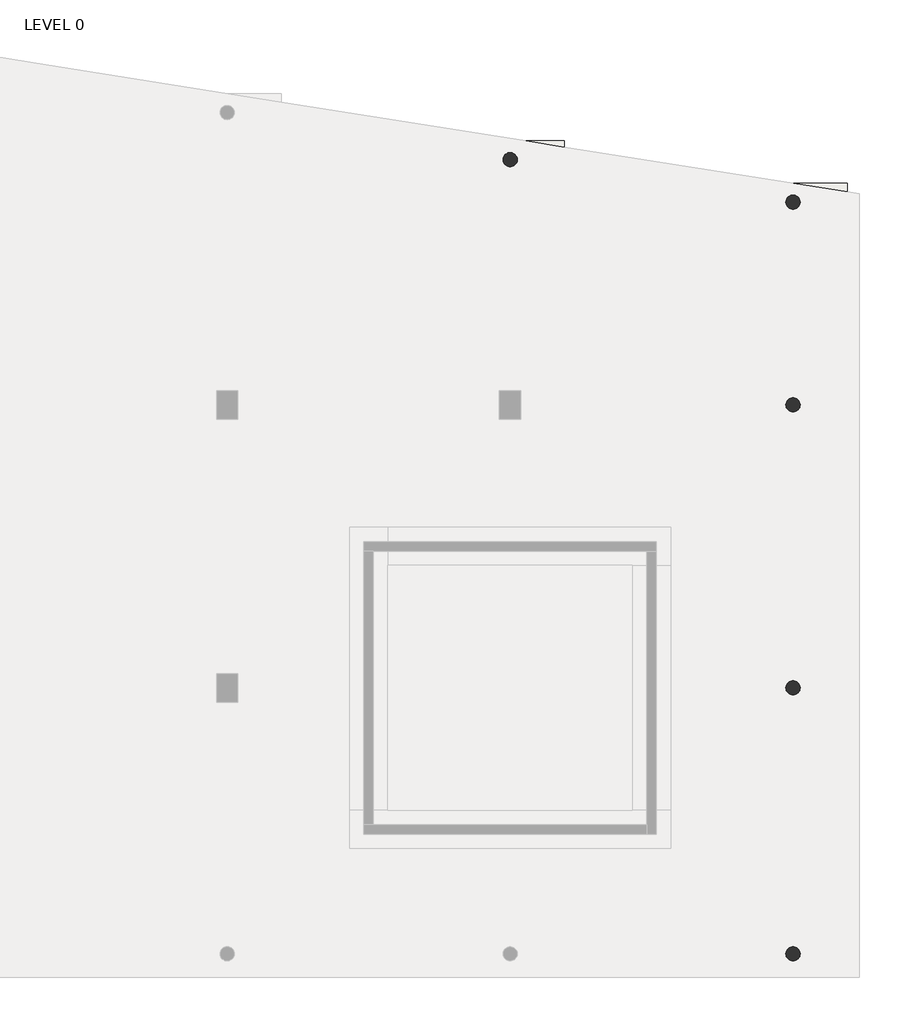
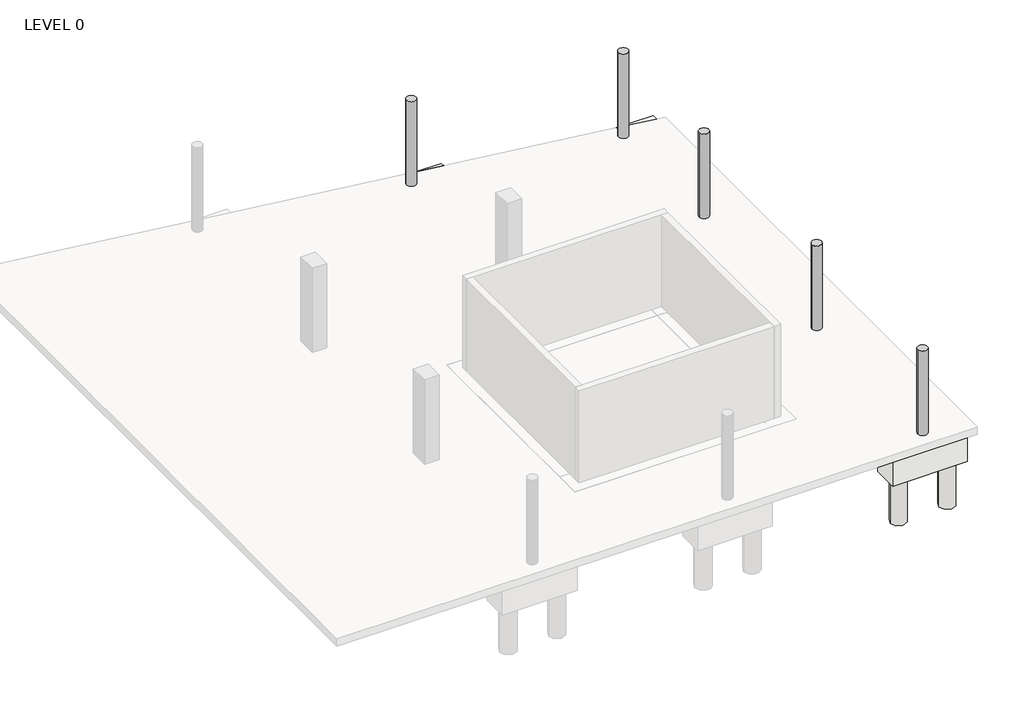
# One storey, part 3 of 3: 17 slabs, 5 columns.
"""IFC4 building model written with IfcOpenShell, lengths in millimetres."""

from ifc_helpers import new_model, si_unit, point, frame, frame_2d, origin, origin_with_axes, place, context, project, spatial, polyline, circle_curve, trimmed, segment, composite_curve, outline, extrude, element, save
from ifc_brep_helpers import plane_surface, cylinder_surface, revolved_surface, advanced_brep

model = new_model("IFC4")

# Units and contexts
model_context = context("Model", 3, world=origin())
ifc_project = project(units=[si_unit("LENGTHUNIT", "METRE", prefix="MILLI")], contexts=[model_context])

# Site, building, storey
site = spatial("IfcSite", under=ifc_project)
building = spatial("IfcBuilding", under=site)
storey = spatial("IfcBuildingStorey", under=building, Name="LEVEL 0", Elevation=0.0)

# Columns
placement = place(None, origin())
element("IfcColumn", 1, ObjectType="BHm_StructuralColumns_ConcreteRound : 300 Ø RC COL", at=placement, inside=storey, context=model_context, shape_type="SweptSolid", body=[
    extrude(outline(composite_curve([segment(trimmed(circle_curve(frame_2d((924.8319731, 14640.7845261)), 150.0), [point((774.8319731, 14640.7845261))], [point((1074.8319731, 14640.7845261))], False, "CARTESIAN"), True, "CONTINUOUS"), segment(trimmed(circle_curve(frame_2d((924.8319731, 14640.7845261)), 150.0), [point((1074.8319731, 14640.7845261))], [point((774.8319731, 14640.7845261))], False, "CARTESIAN"), True, "CONTINUOUS")], self_intersect=False)), origin_with_axes(), (0.0, 0.0, 1.0), 2750.0),
])
element("IfcColumn", 2, ObjectType="BHm_StructuralColumns_ConcreteRound : 300 Ø RC COL", at=placement, inside=storey, context=model_context, shape_type="SweptSolid", body=[
    extrude(outline(composite_curve([segment(trimmed(circle_curve(frame_2d((924.8319731, 8640.7845261)), 150.0), [point((774.8319731, 8640.7845261))], [point((1074.8319731, 8640.7845261))], False, "CARTESIAN"), True, "CONTINUOUS"), segment(trimmed(circle_curve(frame_2d((924.8319731, 8640.7845261)), 150.0), [point((1074.8319731, 8640.7845261))], [point((774.8319731, 8640.7845261))], False, "CARTESIAN"), True, "CONTINUOUS")], self_intersect=False)), origin_with_axes(), (0.0, 0.0, 1.0), 2750.0),
])
element("IfcColumn", 3, ObjectType="BHm_StructuralColumns_ConcreteRound : 300 Ø RC COL", at=placement, inside=storey, context=model_context, shape_type="SweptSolid", body=[
    extrude(outline(composite_curve([segment(trimmed(circle_curve(frame_2d((924.8319731, 3000.0)), 150.0), [point((774.8319731, 3000.0))], [point((1074.8319731, 3000.0))], False, "CARTESIAN"), True, "CONTINUOUS"), segment(trimmed(circle_curve(frame_2d((924.8319731, 3000.0)), 150.0), [point((1074.8319731, 3000.0))], [point((774.8319731, 3000.0))], False, "CARTESIAN"), True, "CONTINUOUS")], self_intersect=False)), origin_with_axes(), (0.0, 0.0, 1.0), 2750.0),
])
element("IfcColumn", 4, ObjectType="BHm_StructuralColumns_ConcreteRound : 300 Ø RC COL", at=placement, inside=storey, context=model_context, shape_type="SweptSolid", body=[
    extrude(outline(composite_curve([segment(trimmed(circle_curve(frame_2d((-5075.1680269, 19840.7845261)), 150.0), [point((-5225.1680269, 19840.7845261))], [point((-4925.1680269, 19840.7845261))], False, "CARTESIAN"), True, "CONTINUOUS"), segment(trimmed(circle_curve(frame_2d((-5075.1680269, 19840.7845261)), 150.0), [point((-4925.1680269, 19840.7845261))], [point((-5225.1680269, 19840.7845261))], False, "CARTESIAN"), True, "CONTINUOUS")], self_intersect=False)), origin_with_axes(), (0.0, 0.0, 1.0), 2750.0),
])
element("IfcColumn", 5, ObjectType="BHm_StructuralColumns_ConcreteRound : 300 Ø RC COL", at=placement, inside=storey, context=model_context, shape_type="SweptSolid", body=[
    extrude(outline(composite_curve([segment(trimmed(circle_curve(frame_2d((924.8319731, 18940.7845261)), 150.0), [point((774.8319731, 18940.7845261))], [point((1074.8319731, 18940.7845261))], False, "CARTESIAN"), True, "CONTINUOUS"), segment(trimmed(circle_curve(frame_2d((924.8319731, 18940.7845261)), 150.0), [point((1074.8319731, 18940.7845261))], [point((774.8319731, 18940.7845261))], False, "CARTESIAN"), True, "CONTINUOUS")], self_intersect=False)), origin_with_axes(), (0.0, 0.0, 1.0), 2750.0),
])

# Slabs
element("IfcSlab", 6, ObjectType="BHm_StructuralFoundations_RC-2PileCap : 500Ø R.C. 2-PILE CAP", at=placement, inside=storey, context=model_context, shape_type="AdvancedBrep", body=[
    advanced_brep(
    [(2074.8319731, 3400.0, -1100.0), (2074.8319731, 2600.0, -1100.0), (-225.1680269, 2600.0, -1100.0), (-225.1680269, 3400.0, -1100.0), (-75.1680269, 3000.0, -1100.0), (424.8319731, 3000.0, -1100.0), (1424.8319731, 3000.0, -1100.0), (1924.8319731, 3000.0, -1100.0), (-225.1680269, 3400.0, -250.0), (2074.8319731, 3400.0, -250.0), (-225.1680269, 2600.0, -250.0), (2074.8319731, 2600.0, -250.0), (1424.8319731, 3000.0, -1025.0), (1924.8319731, 3000.0, -1025.0), (-75.1680269, 3000.0, -1025.0), (424.8319731, 3000.0, -1025.0)],
    [
        (0, 1),
        (1, 2),
        (2, 3),
        (3, 0),
        (4, 5, circle_curve(frame((174.8319731, 3000.0, -1100.0), z_axis=(0.0, 0.0, 1.0), x_axis=(1.0, 0.0, 0.0)), 250.0)),
        (5, 4, circle_curve(frame((174.8319731, 3000.0, -1100.0), z_axis=(0.0, 0.0, 1.0), x_axis=(1.0, 0.0, 0.0)), 250.0)),
        (6, 7, circle_curve(frame((1674.8319731, 3000.0, -1100.0), z_axis=(0.0, 0.0, 1.0), x_axis=(1.0, 0.0, 0.0)), 250.0)),
        (7, 6, circle_curve(frame((1674.8319731, 3000.0, -1100.0), z_axis=(0.0, 0.0, 1.0), x_axis=(1.0, 0.0, 0.0)), 250.0)),
        (3, 8),
        (8, 9),
        (9, 0),
        (2, 10),
        (10, 8),
        (1, 11),
        (11, 10),
        (9, 11),
        (12, 13, circle_curve(frame((1674.8319731, 3000.0, -1025.0), z_axis=(0.0, 0.0, -1.0), x_axis=(1.0, 0.0, 0.0)), 250.0)),
        (13, 12, circle_curve(frame((1674.8319731, 3000.0, -1025.0), z_axis=(0.0, 0.0, -1.0), x_axis=(1.0, 0.0, 0.0)), 250.0)),
        (4, 14),
        (14, 15, circle_curve(frame((174.8319731, 3000.0, -1025.0), z_axis=(0.0, 0.0, 1.0), x_axis=(1.0, 0.0, 0.0)), 250.0)),
        (15, 5),
        (15, 14, circle_curve(frame((174.8319731, 3000.0, -1025.0), z_axis=(0.0, 0.0, 1.0), x_axis=(1.0, 0.0, 0.0)), 250.0)),
        (6, 12),
        (13, 7),
    ],
    [
        plane_surface(frame((-225.1680269, 3400.0, -1100.0), z_axis=(0.0, 0.0, -1.0), x_axis=(1.0, 0.0, 0.0))),
        plane_surface(frame((2074.8319731, 3400.0, 0.0), z_axis=(0.0, 1.0, 0.0), x_axis=(0.0, 0.0, -1.0))),
        plane_surface(frame((-225.1680269, 3400.0, 0.0), z_axis=(-1.0, 0.0, 0.0), x_axis=(0.0, 0.0, -1.0))),
        plane_surface(frame((-225.1680269, 2600.0, 0.0), z_axis=(0.0, -1.0, 0.0), x_axis=(0.0, 0.0, -1.0))),
        plane_surface(frame((2074.8319731, 2600.0, 0.0), z_axis=(1.0, 0.0, 0.0), x_axis=(0.0, 0.0, -1.0))),
        plane_surface(frame((424.8319731, 3000.0, -1025.0), z_axis=(0.0, 0.0, -1.0), x_axis=(0.0, 1.0, 0.0))),
        revolved_surface(polyline([(424.8319731, 3000.0, -1025.0), (424.8319731, 3000.0, -1100.0)]), (174.8319731, 3000.0, -1100.0), (0.0, 0.0, 1.0)),
        revolved_surface(polyline([(1924.8319731, 3000.0, -1025.0), (1924.8319731, 3000.0, -1100.0)]), (1674.8319731, 3000.0, 0.0), (0.0, 0.0, 1.0)),
        plane_surface(frame((2324.8319731, 15140.7845261, -250.0), z_axis=(0.0, 0.0, 1.0), x_axis=(0.0, -1.0, 0.0))),
    ],
    [
        (0, [[1, 2, 3, 4], [5, 6], [7, 8]]),
        (1, [[-4, 9, 10, 11]]),
        (2, [[-3, 12, 13, -9]]),
        (3, [[-2, 14, 15, -12]]),
        (4, [[-1, -11, 16, -14]]),
        (5, [[17, 18]]),
        (6, [[-5, 19, 20, 21]]),
        (6, [[-6, -21, 22, -19]]),
        (7, [[-7, 23, -18, 24]]),
        (7, [[-8, -24, -17, -23]]),
        (8, [[-10, -13, -15, -16]]),
        (5, [[-22, -20]]),
    ],
),
])
element("IfcSlab", 7, ObjectType="BHm_StructuralFoundations_RC-Pile : 500Ø R.C. PILE", at=placement, inside=storey, context=model_context, shape_type="AdvancedBrep", body=[
    advanced_brep(
    [(-75.1680269, 3000.0, -1025.0), (424.8319731, 3000.0, -1025.0), (-75.1680269, 3000.0, -2600.0), (424.8319731, 3000.0, -2600.0), (-75.1680269, 3000.0, -1100.0), (424.8319731, 3000.0, -1100.0)],
    [
        (0, 1, circle_curve(frame((174.8319731, 3000.0, -1025.0), z_axis=(0.0, 0.0, 1.0), x_axis=(1.0, 0.0, 0.0)), 250.0)),
        (1, 0, circle_curve(frame((174.8319731, 3000.0, -1025.0), z_axis=(0.0, 0.0, 1.0), x_axis=(1.0, 0.0, 0.0)), 250.0)),
        (2, 3, circle_curve(frame((174.8319731, 3000.0, -2600.0), z_axis=(0.0, 0.0, -1.0), x_axis=(1.0, 0.0, 0.0)), 250.0)),
        (3, 2, circle_curve(frame((174.8319731, 3000.0, -2600.0), z_axis=(0.0, 0.0, -1.0), x_axis=(1.0, 0.0, 0.0)), 250.0)),
        (0, 4),
        (4, 2),
        (3, 5),
        (5, 1),
    ],
    [
        plane_surface(frame((424.8319731, 3000.0, -1025.0), z_axis=(0.0, 0.0, 1.0), x_axis=(0.0, 1.0, 0.0))),
        plane_surface(frame((424.8319731, 3000.0, -2600.0), z_axis=(0.0, 0.0, -1.0), x_axis=(0.0, -1.0, 0.0))),
        cylinder_surface(frame((174.8319731, 3000.0, -2600.0), z_axis=(0.0, 0.0, 1.0), x_axis=(1.0, 0.0, 0.0)), 250.0),
    ],
    [
        (0, [[1, 2]]),
        (1, [[3, 4]]),
        (2, [[-1, 5, 6, -4, 7, 8]]),
        (2, [[-2, -8, -7, -3, -6, -5]]),
    ],
),
])
element("IfcSlab", 8, ObjectType="BHm_StructuralFoundations_RC-Pile : 500Ø R.C. PILE", at=placement, inside=storey, context=model_context, shape_type="AdvancedBrep", body=[
    advanced_brep(
    [(1424.8319731, 3000.0, -1025.0), (1924.8319731, 3000.0, -1025.0), (1424.8319731, 3000.0, -2600.0), (1924.8319731, 3000.0, -2600.0), (1424.8319731, 3000.0, -1100.0), (1924.8319731, 3000.0, -1100.0)],
    [
        (0, 1, circle_curve(frame((1674.8319731, 3000.0, -1025.0), z_axis=(0.0, 0.0, 1.0), x_axis=(1.0, 0.0, 0.0)), 250.0)),
        (1, 0, circle_curve(frame((1674.8319731, 3000.0, -1025.0), z_axis=(0.0, 0.0, 1.0), x_axis=(1.0, 0.0, 0.0)), 250.0)),
        (2, 3, circle_curve(frame((1674.8319731, 3000.0, -2600.0), z_axis=(0.0, 0.0, -1.0), x_axis=(1.0, 0.0, 0.0)), 250.0)),
        (3, 2, circle_curve(frame((1674.8319731, 3000.0, -2600.0), z_axis=(0.0, 0.0, -1.0), x_axis=(1.0, 0.0, 0.0)), 250.0)),
        (0, 4),
        (4, 2),
        (3, 5),
        (5, 1),
    ],
    [
        plane_surface(frame((1924.8319731, 3000.0, -1025.0), z_axis=(0.0, 0.0, 1.0), x_axis=(0.0, 1.0, 0.0))),
        plane_surface(frame((1924.8319731, 3000.0, -2600.0), z_axis=(0.0, 0.0, -1.0), x_axis=(0.0, -1.0, 0.0))),
        cylinder_surface(frame((1674.8319731, 3000.0, -2600.0), z_axis=(0.0, 0.0, 1.0), x_axis=(1.0, 0.0, 0.0)), 250.0),
    ],
    [
        (0, [[1, 2]]),
        (1, [[3, 4]]),
        (2, [[-1, 5, 6, -4, 7, 8]]),
        (2, [[-2, -8, -7, -3, -6, -5]]),
    ],
),
])
element("IfcSlab", 9, ObjectType="BHm_StructuralFoundations_RC-2PileCap : 500Ø R.C. 2-PILE CAP", at=placement, inside=storey, context=model_context, shape_type="AdvancedBrep", body=[
    advanced_brep(
    [(2074.8319731, 9040.7845261, -1100.0), (2074.8319731, 8240.7845261, -1100.0), (-225.1680269, 8240.7845261, -1100.0), (-225.1680269, 9040.7845261, -1100.0), (-75.1680269, 8640.7845261, -1100.0), (424.8319731, 8640.7845261, -1100.0), (1424.8319731, 8640.7845261, -1100.0), (1924.8319731, 8640.7845261, -1100.0), (-225.1680269, 9040.7845261, -250.0), (2074.8319731, 9040.7845261, -250.0), (-225.1680269, 8240.7845261, -250.0), (2074.8319731, 8240.7845261, -250.0), (1424.8319731, 8640.7845261, -1025.0), (1924.8319731, 8640.7845261, -1025.0), (-75.1680269, 8640.7845261, -1025.0), (424.8319731, 8640.7845261, -1025.0)],
    [
        (0, 1),
        (1, 2),
        (2, 3),
        (3, 0),
        (4, 5, circle_curve(frame((174.8319731, 8640.7845261, -1100.0), z_axis=(0.0, 0.0, 1.0), x_axis=(1.0, 0.0, 0.0)), 250.0)),
        (5, 4, circle_curve(frame((174.8319731, 8640.7845261, -1100.0), z_axis=(0.0, 0.0, 1.0), x_axis=(1.0, 0.0, 0.0)), 250.0)),
        (6, 7, circle_curve(frame((1674.8319731, 8640.7845261, -1100.0), z_axis=(0.0, 0.0, 1.0), x_axis=(1.0, 0.0, 0.0)), 250.0)),
        (7, 6, circle_curve(frame((1674.8319731, 8640.7845261, -1100.0), z_axis=(0.0, 0.0, 1.0), x_axis=(1.0, 0.0, 0.0)), 250.0)),
        (3, 8),
        (8, 9),
        (9, 0),
        (2, 10),
        (10, 8),
        (1, 11),
        (11, 10),
        (9, 11),
        (12, 13, circle_curve(frame((1674.8319731, 8640.7845261, -1025.0), z_axis=(0.0, 0.0, -1.0), x_axis=(1.0, 0.0, 0.0)), 250.0)),
        (13, 12, circle_curve(frame((1674.8319731, 8640.7845261, -1025.0), z_axis=(0.0, 0.0, -1.0), x_axis=(1.0, 0.0, 0.0)), 250.0)),
        (4, 14),
        (14, 15, circle_curve(frame((174.8319731, 8640.7845261, -1025.0), z_axis=(0.0, 0.0, 1.0), x_axis=(1.0, 0.0, 0.0)), 250.0)),
        (15, 5),
        (15, 14, circle_curve(frame((174.8319731, 8640.7845261, -1025.0), z_axis=(0.0, 0.0, 1.0), x_axis=(1.0, 0.0, 0.0)), 250.0)),
        (6, 12),
        (13, 7),
    ],
    [
        plane_surface(frame((-225.1680269, 9040.7845261, -1100.0), z_axis=(0.0, 0.0, -1.0), x_axis=(1.0, 0.0, 0.0))),
        plane_surface(frame((2074.8319731, 9040.7845261, 0.0), z_axis=(0.0, 1.0, 0.0), x_axis=(0.0, 0.0, -1.0))),
        plane_surface(frame((-225.1680269, 9040.7845261, 0.0), z_axis=(-1.0, 0.0, 0.0), x_axis=(0.0, 0.0, -1.0))),
        plane_surface(frame((-225.1680269, 8240.7845261, 0.0), z_axis=(0.0, -1.0, 0.0), x_axis=(0.0, 0.0, -1.0))),
        plane_surface(frame((2074.8319731, 8240.7845261, 0.0), z_axis=(1.0, 0.0, 0.0), x_axis=(0.0, 0.0, -1.0))),
        plane_surface(frame((424.8319731, 8640.7845261, -1025.0), z_axis=(0.0, 0.0, -1.0), x_axis=(0.0, 1.0, 0.0))),
        revolved_surface(polyline([(424.8319731, 8640.7845261, -1025.0), (424.8319731, 8640.7845261, -1100.0)]), (174.8319731, 8640.7845261, -1100.0), (0.0, 0.0, 1.0)),
        revolved_surface(polyline([(1924.8319731, 8640.7845261, -1025.0), (1924.8319731, 8640.7845261, -1100.0)]), (1674.8319731, 8640.7845261, 0.0), (0.0, 0.0, 1.0)),
        plane_surface(frame((2324.8319731, 15140.7845261, -250.0), z_axis=(0.0, 0.0, 1.0), x_axis=(0.0, -1.0, 0.0))),
    ],
    [
        (0, [[1, 2, 3, 4], [5, 6], [7, 8]]),
        (1, [[-4, 9, 10, 11]]),
        (2, [[-3, 12, 13, -9]]),
        (3, [[-2, 14, 15, -12]]),
        (4, [[-1, -11, 16, -14]]),
        (5, [[17, 18]]),
        (6, [[-5, 19, 20, 21]]),
        (6, [[-6, -21, 22, -19]]),
        (7, [[-7, 23, -18, 24]]),
        (7, [[-8, -24, -17, -23]]),
        (8, [[-10, -13, -15, -16]]),
        (5, [[-22, -20]]),
    ],
),
])
element("IfcSlab", 10, ObjectType="BHm_StructuralFoundations_RC-Pile : 500Ø R.C. PILE", at=placement, inside=storey, context=model_context, shape_type="AdvancedBrep", body=[
    advanced_brep(
    [(-75.1680269, 8640.7845261, -1025.0), (424.8319731, 8640.7845261, -1025.0), (-75.1680269, 8640.7845261, -2600.0), (424.8319731, 8640.7845261, -2600.0), (-75.1680269, 8640.7845261, -1100.0), (424.8319731, 8640.7845261, -1100.0)],
    [
        (0, 1, circle_curve(frame((174.8319731, 8640.7845261, -1025.0), z_axis=(0.0, 0.0, 1.0), x_axis=(1.0, 0.0, 0.0)), 250.0)),
        (1, 0, circle_curve(frame((174.8319731, 8640.7845261, -1025.0), z_axis=(0.0, 0.0, 1.0), x_axis=(1.0, 0.0, 0.0)), 250.0)),
        (2, 3, circle_curve(frame((174.8319731, 8640.7845261, -2600.0), z_axis=(0.0, 0.0, -1.0), x_axis=(1.0, 0.0, 0.0)), 250.0)),
        (3, 2, circle_curve(frame((174.8319731, 8640.7845261, -2600.0), z_axis=(0.0, 0.0, -1.0), x_axis=(1.0, 0.0, 0.0)), 250.0)),
        (0, 4),
        (4, 2),
        (3, 5),
        (5, 1),
    ],
    [
        plane_surface(frame((424.8319731, 8640.7845261, -1025.0), z_axis=(0.0, 0.0, 1.0), x_axis=(0.0, 1.0, 0.0))),
        plane_surface(frame((424.8319731, 8640.7845261, -2600.0), z_axis=(0.0, 0.0, -1.0), x_axis=(0.0, -1.0, 0.0))),
        cylinder_surface(frame((174.8319731, 8640.7845261, -2600.0), z_axis=(0.0, 0.0, 1.0), x_axis=(1.0, 0.0, 0.0)), 250.0),
    ],
    [
        (0, [[1, 2]]),
        (1, [[3, 4]]),
        (2, [[-1, 5, 6, -4, 7, 8]]),
        (2, [[-2, -8, -7, -3, -6, -5]]),
    ],
),
])
element("IfcSlab", 11, ObjectType="BHm_StructuralFoundations_RC-Pile : 500Ø R.C. PILE", at=placement, inside=storey, context=model_context, shape_type="AdvancedBrep", body=[
    advanced_brep(
    [(1424.8319731, 8640.7845261, -1025.0), (1924.8319731, 8640.7845261, -1025.0), (1424.8319731, 8640.7845261, -2600.0), (1924.8319731, 8640.7845261, -2600.0), (1424.8319731, 8640.7845261, -1100.0), (1924.8319731, 8640.7845261, -1100.0)],
    [
        (0, 1, circle_curve(frame((1674.8319731, 8640.7845261, -1025.0), z_axis=(0.0, 0.0, 1.0), x_axis=(1.0, 0.0, 0.0)), 250.0)),
        (1, 0, circle_curve(frame((1674.8319731, 8640.7845261, -1025.0), z_axis=(0.0, 0.0, 1.0), x_axis=(1.0, 0.0, 0.0)), 250.0)),
        (2, 3, circle_curve(frame((1674.8319731, 8640.7845261, -2600.0), z_axis=(0.0, 0.0, -1.0), x_axis=(1.0, 0.0, 0.0)), 250.0)),
        (3, 2, circle_curve(frame((1674.8319731, 8640.7845261, -2600.0), z_axis=(0.0, 0.0, -1.0), x_axis=(1.0, 0.0, 0.0)), 250.0)),
        (0, 4),
        (4, 2),
        (3, 5),
        (5, 1),
    ],
    [
        plane_surface(frame((1924.8319731, 8640.7845261, -1025.0), z_axis=(0.0, 0.0, 1.0), x_axis=(0.0, 1.0, 0.0))),
        plane_surface(frame((1924.8319731, 8640.7845261, -2600.0), z_axis=(0.0, 0.0, -1.0), x_axis=(0.0, -1.0, 0.0))),
        cylinder_surface(frame((1674.8319731, 8640.7845261, -2600.0), z_axis=(0.0, 0.0, 1.0), x_axis=(1.0, 0.0, 0.0)), 250.0),
    ],
    [
        (0, [[1, 2]]),
        (1, [[3, 4]]),
        (2, [[-1, 5, 6, -4, 7, 8]]),
        (2, [[-2, -8, -7, -3, -6, -5]]),
    ],
),
])
element("IfcSlab", 12, ObjectType="BHm_StructuralFoundations_RC-2PileCap : 500Ø R.C. 2-PILE CAP", at=placement, inside=storey, context=model_context, shape_type="AdvancedBrep", body=[
    advanced_brep(
    [(2074.8319731, 15040.7845261, -1100.0), (2074.8319731, 14240.7845261, -1100.0), (-225.1680269, 14240.7845261, -1100.0), (-225.1680269, 15040.7845261, -1100.0), (-75.1680269, 14640.7845261, -1100.0), (424.8319731, 14640.7845261, -1100.0), (1424.8319731, 14640.7845261, -1100.0), (1924.8319731, 14640.7845261, -1100.0), (-225.1680269, 15040.7845261, -250.0), (2074.8319731, 15040.7845261, -250.0), (-225.1680269, 14240.7845261, -250.0), (2074.8319731, 14240.7845261, -250.0), (1424.8319731, 14640.7845261, -1025.0), (1924.8319731, 14640.7845261, -1025.0), (-75.1680269, 14640.7845261, -1025.0), (424.8319731, 14640.7845261, -1025.0)],
    [
        (0, 1),
        (1, 2),
        (2, 3),
        (3, 0),
        (4, 5, circle_curve(frame((174.8319731, 14640.7845261, -1100.0), z_axis=(0.0, 0.0, 1.0), x_axis=(1.0, 0.0, 0.0)), 250.0)),
        (5, 4, circle_curve(frame((174.8319731, 14640.7845261, -1100.0), z_axis=(0.0, 0.0, 1.0), x_axis=(1.0, 0.0, 0.0)), 250.0)),
        (6, 7, circle_curve(frame((1674.8319731, 14640.7845261, -1100.0), z_axis=(0.0, 0.0, 1.0), x_axis=(1.0, 0.0, 0.0)), 250.0)),
        (7, 6, circle_curve(frame((1674.8319731, 14640.7845261, -1100.0), z_axis=(0.0, 0.0, 1.0), x_axis=(1.0, 0.0, 0.0)), 250.0)),
        (3, 8),
        (8, 9),
        (9, 0),
        (2, 10),
        (10, 8),
        (1, 11),
        (11, 10),
        (9, 11),
        (12, 13, circle_curve(frame((1674.8319731, 14640.7845261, -1025.0), z_axis=(0.0, 0.0, -1.0), x_axis=(1.0, 0.0, 0.0)), 250.0)),
        (13, 12, circle_curve(frame((1674.8319731, 14640.7845261, -1025.0), z_axis=(0.0, 0.0, -1.0), x_axis=(1.0, 0.0, 0.0)), 250.0)),
        (4, 14),
        (14, 15, circle_curve(frame((174.8319731, 14640.7845261, -1025.0), z_axis=(0.0, 0.0, 1.0), x_axis=(1.0, 0.0, 0.0)), 250.0)),
        (15, 5),
        (15, 14, circle_curve(frame((174.8319731, 14640.7845261, -1025.0), z_axis=(0.0, 0.0, 1.0), x_axis=(1.0, 0.0, 0.0)), 250.0)),
        (6, 12),
        (13, 7),
    ],
    [
        plane_surface(frame((-225.1680269, 15040.7845261, -1100.0), z_axis=(0.0, 0.0, -1.0), x_axis=(1.0, 0.0, 0.0))),
        plane_surface(frame((2074.8319731, 15040.7845261, 0.0), z_axis=(0.0, 1.0, 0.0), x_axis=(0.0, 0.0, -1.0))),
        plane_surface(frame((-225.1680269, 15040.7845261, 0.0), z_axis=(-1.0, 0.0, 0.0), x_axis=(0.0, 0.0, -1.0))),
        plane_surface(frame((-225.1680269, 14240.7845261, 0.0), z_axis=(0.0, -1.0, 0.0), x_axis=(0.0, 0.0, -1.0))),
        plane_surface(frame((2074.8319731, 14240.7845261, 0.0), z_axis=(1.0, 0.0, 0.0), x_axis=(0.0, 0.0, -1.0))),
        plane_surface(frame((424.8319731, 14640.7845261, -1025.0), z_axis=(0.0, 0.0, -1.0), x_axis=(0.0, 1.0, 0.0))),
        revolved_surface(polyline([(424.8319731, 14640.7845261, -1025.0), (424.8319731, 14640.7845261, -1100.0)]), (174.8319731, 14640.7845261, -1100.0), (0.0, 0.0, 1.0)),
        revolved_surface(polyline([(1924.8319731, 14640.7845261, -1025.0), (1924.8319731, 14640.7845261, -1100.0)]), (1674.8319731, 14640.7845261, 0.0), (0.0, 0.0, 1.0)),
        plane_surface(frame((2324.8319731, 15140.7845261, -250.0), z_axis=(0.0, 0.0, 1.0), x_axis=(0.0, -1.0, 0.0))),
    ],
    [
        (0, [[1, 2, 3, 4], [5, 6], [7, 8]]),
        (1, [[-4, 9, 10, 11]]),
        (2, [[-3, 12, 13, -9]]),
        (3, [[-2, 14, 15, -12]]),
        (4, [[-1, -11, 16, -14]]),
        (5, [[17, 18]]),
        (6, [[-5, 19, 20, 21]]),
        (6, [[-6, -21, 22, -19]]),
        (7, [[-7, 23, -18, 24]]),
        (7, [[-8, -24, -17, -23]]),
        (8, [[-10, -13, -15, -16]]),
        (5, [[-22, -20]]),
    ],
),
])
element("IfcSlab", 13, ObjectType="BHm_StructuralFoundations_RC-Pile : 500Ø R.C. PILE", at=placement, inside=storey, context=model_context, shape_type="AdvancedBrep", body=[
    advanced_brep(
    [(-75.1680269, 14640.7845261, -1025.0), (424.8319731, 14640.7845261, -1025.0), (-75.1680269, 14640.7845261, -2600.0), (424.8319731, 14640.7845261, -2600.0), (-75.1680269, 14640.7845261, -1100.0), (424.8319731, 14640.7845261, -1100.0)],
    [
        (0, 1, circle_curve(frame((174.8319731, 14640.7845261, -1025.0), z_axis=(0.0, 0.0, 1.0), x_axis=(1.0, 0.0, 0.0)), 250.0)),
        (1, 0, circle_curve(frame((174.8319731, 14640.7845261, -1025.0), z_axis=(0.0, 0.0, 1.0), x_axis=(1.0, 0.0, 0.0)), 250.0)),
        (2, 3, circle_curve(frame((174.8319731, 14640.7845261, -2600.0), z_axis=(0.0, 0.0, -1.0), x_axis=(1.0, 0.0, 0.0)), 250.0)),
        (3, 2, circle_curve(frame((174.8319731, 14640.7845261, -2600.0), z_axis=(0.0, 0.0, -1.0), x_axis=(1.0, 0.0, 0.0)), 250.0)),
        (0, 4),
        (4, 2),
        (3, 5),
        (5, 1),
    ],
    [
        plane_surface(frame((424.8319731, 14640.7845261, -1025.0), z_axis=(0.0, 0.0, 1.0), x_axis=(0.0, 1.0, 0.0))),
        plane_surface(frame((424.8319731, 14640.7845261, -2600.0), z_axis=(0.0, 0.0, -1.0), x_axis=(0.0, -1.0, 0.0))),
        cylinder_surface(frame((174.8319731, 14640.7845261, -2600.0), z_axis=(0.0, 0.0, 1.0), x_axis=(1.0, 0.0, 0.0)), 250.0),
    ],
    [
        (0, [[1, 2]]),
        (1, [[3, 4]]),
        (2, [[-1, 5, 6, -4, 7, 8]]),
        (2, [[-2, -8, -7, -3, -6, -5]]),
    ],
),
])
element("IfcSlab", 14, ObjectType="BHm_StructuralFoundations_RC-Pile : 500Ø R.C. PILE", at=placement, inside=storey, context=model_context, shape_type="AdvancedBrep", body=[
    advanced_brep(
    [(1424.8319731, 14640.7845261, -1025.0), (1924.8319731, 14640.7845261, -1025.0), (1424.8319731, 14640.7845261, -2600.0), (1924.8319731, 14640.7845261, -2600.0), (1424.8319731, 14640.7845261, -1100.0), (1924.8319731, 14640.7845261, -1100.0)],
    [
        (0, 1, circle_curve(frame((1674.8319731, 14640.7845261, -1025.0), z_axis=(0.0, 0.0, 1.0), x_axis=(1.0, 0.0, 0.0)), 250.0)),
        (1, 0, circle_curve(frame((1674.8319731, 14640.7845261, -1025.0), z_axis=(0.0, 0.0, 1.0), x_axis=(1.0, 0.0, 0.0)), 250.0)),
        (2, 3, circle_curve(frame((1674.8319731, 14640.7845261, -2600.0), z_axis=(0.0, 0.0, -1.0), x_axis=(1.0, 0.0, 0.0)), 250.0)),
        (3, 2, circle_curve(frame((1674.8319731, 14640.7845261, -2600.0), z_axis=(0.0, 0.0, -1.0), x_axis=(1.0, 0.0, 0.0)), 250.0)),
        (0, 4),
        (4, 2),
        (3, 5),
        (5, 1),
    ],
    [
        plane_surface(frame((1924.8319731, 14640.7845261, -1025.0), z_axis=(0.0, 0.0, 1.0), x_axis=(0.0, 1.0, 0.0))),
        plane_surface(frame((1924.8319731, 14640.7845261, -2600.0), z_axis=(0.0, 0.0, -1.0), x_axis=(0.0, -1.0, 0.0))),
        cylinder_surface(frame((1674.8319731, 14640.7845261, -2600.0), z_axis=(0.0, 0.0, 1.0), x_axis=(1.0, 0.0, 0.0)), 250.0),
    ],
    [
        (0, [[1, 2]]),
        (1, [[3, 4]]),
        (2, [[-1, 5, 6, -4, 7, 8]]),
        (2, [[-2, -8, -7, -3, -6, -5]]),
    ],
),
])
element("IfcSlab", 15, ObjectType="BHm_StructuralFoundations_RC-Pile : 500Ø R.C. PILE", at=placement, inside=storey, context=model_context, shape_type="AdvancedBrep", body=[
    advanced_brep(
    [(-12075.1680269, 20840.7845261, -1025.0), (-11575.1680269, 20840.7845261, -1025.0), (-12075.1680269, 20840.7845261, -2600.0), (-11575.1680269, 20840.7845261, -2600.0), (-12075.1680269, 20840.7845261, -1100.0), (-11575.1680269, 20840.7845261, -1100.0)],
    [
        (0, 1, circle_curve(frame((-11825.1680269, 20840.7845261, -1025.0), z_axis=(0.0, 0.0, 1.0), x_axis=(1.0, 0.0, 0.0)), 250.0)),
        (1, 0, circle_curve(frame((-11825.1680269, 20840.7845261, -1025.0), z_axis=(0.0, 0.0, 1.0), x_axis=(1.0, 0.0, 0.0)), 250.0)),
        (2, 3, circle_curve(frame((-11825.1680269, 20840.7845261, -2600.0), z_axis=(0.0, 0.0, -1.0), x_axis=(1.0, 0.0, 0.0)), 250.0)),
        (3, 2, circle_curve(frame((-11825.1680269, 20840.7845261, -2600.0), z_axis=(0.0, 0.0, -1.0), x_axis=(1.0, 0.0, 0.0)), 250.0)),
        (0, 4),
        (4, 2),
        (3, 5),
        (5, 1),
    ],
    [
        plane_surface(frame((-11575.1680269, 20840.7845261, -1025.0), z_axis=(0.0, 0.0, 1.0), x_axis=(0.0, 1.0, 0.0))),
        plane_surface(frame((-11575.1680269, 20840.7845261, -2600.0), z_axis=(0.0, 0.0, -1.0), x_axis=(0.0, -1.0, 0.0))),
        cylinder_surface(frame((-11825.1680269, 20840.7845261, -2600.0), z_axis=(0.0, 0.0, 1.0), x_axis=(1.0, 0.0, 0.0)), 250.0),
    ],
    [
        (0, [[1, 2]]),
        (1, [[3, 4]]),
        (2, [[-1, 5, 6, -4, 7, 8]]),
        (2, [[-2, -8, -7, -3, -6, -5]]),
    ],
),
])
element("IfcSlab", 16, ObjectType="BHm_StructuralFoundations_RC-Pile : 500Ø R.C. PILE", at=placement, inside=storey, context=model_context, shape_type="AdvancedBrep", body=[
    advanced_brep(
    [(-10575.1680269, 20840.7845261, -1025.0), (-10075.1680269, 20840.7845261, -1025.0), (-10575.1680269, 20840.7845261, -2600.0), (-10075.1680269, 20840.7845261, -2600.0), (-10575.1680269, 20840.7845261, -1100.0), (-10075.1680269, 20840.7845261, -1100.0)],
    [
        (0, 1, circle_curve(frame((-10325.1680269, 20840.7845261, -1025.0), z_axis=(0.0, 0.0, 1.0), x_axis=(1.0, 0.0, 0.0)), 250.0)),
        (1, 0, circle_curve(frame((-10325.1680269, 20840.7845261, -1025.0), z_axis=(0.0, 0.0, 1.0), x_axis=(1.0, 0.0, 0.0)), 250.0)),
        (2, 3, circle_curve(frame((-10325.1680269, 20840.7845261, -2600.0), z_axis=(0.0, 0.0, -1.0), x_axis=(1.0, 0.0, 0.0)), 250.0)),
        (3, 2, circle_curve(frame((-10325.1680269, 20840.7845261, -2600.0), z_axis=(0.0, 0.0, -1.0), x_axis=(1.0, 0.0, 0.0)), 250.0)),
        (0, 4),
        (4, 2),
        (3, 5),
        (5, 1),
    ],
    [
        plane_surface(frame((-10075.1680269, 20840.7845261, -1025.0), z_axis=(0.0, 0.0, 1.0), x_axis=(0.0, 1.0, 0.0))),
        plane_surface(frame((-10075.1680269, 20840.7845261, -2600.0), z_axis=(0.0, 0.0, -1.0), x_axis=(0.0, -1.0, 0.0))),
        cylinder_surface(frame((-10325.1680269, 20840.7845261, -2600.0), z_axis=(0.0, 0.0, 1.0), x_axis=(1.0, 0.0, 0.0)), 250.0),
    ],
    [
        (0, [[1, 2]]),
        (1, [[3, 4]]),
        (2, [[-1, 5, 6, -4, 7, 8]]),
        (2, [[-2, -8, -7, -3, -6, -5]]),
    ],
),
])
element("IfcSlab", 17, ObjectType="BHm_StructuralFoundations_RC-2PileCap : 500Ø R.C. 2-PILE CAP", at=placement, inside=storey, context=model_context, shape_type="AdvancedBrep", body=[
    advanced_brep(
    [(-3925.1680269, 20240.7845261, 0.0), (-4747.6649976, 20240.7845261, 0.0), (-3925.1680269, 20110.5138037, 0.0), (-3925.1680269, 20240.7845261, -1100.0), (-3925.1680269, 19440.7845261, -1100.0), (-6225.1680269, 19440.7845261, -1100.0), (-6225.1680269, 20240.7845261, -1100.0), (-6075.1680269, 19840.7845261, -1100.0), (-5575.1680269, 19840.7845261, -1100.0), (-4575.1680269, 19840.7845261, -1100.0), (-4075.1680269, 19840.7845261, -1100.0), (-6225.1680269, 20240.7845261, -250.0), (-4747.6649976, 20240.7845261, -250.0), (-6225.1680269, 19440.7845261, -250.0), (-3925.1680269, 19440.7845261, -250.0), (-3925.1680269, 20110.5138037, -250.0), (-4575.1680269, 19840.7845261, -1025.0), (-4075.1680269, 19840.7845261, -1025.0), (-6075.1680269, 19840.7845261, -1025.0), (-5575.1680269, 19840.7845261, -1025.0)],
    [
        (0, 1),
        (1, 2),
        (2, 0),
        (3, 4),
        (4, 5),
        (5, 6),
        (6, 3),
        (7, 8, circle_curve(frame((-5825.1680269, 19840.7845261, -1100.0), z_axis=(0.0, 0.0, 1.0), x_axis=(1.0, 0.0, 0.0)), 250.0)),
        (8, 7, circle_curve(frame((-5825.1680269, 19840.7845261, -1100.0), z_axis=(0.0, 0.0, 1.0), x_axis=(1.0, 0.0, 0.0)), 250.0)),
        (9, 10, circle_curve(frame((-4325.1680269, 19840.7845261, -1100.0), z_axis=(0.0, 0.0, 1.0), x_axis=(1.0, 0.0, 0.0)), 250.0)),
        (10, 9, circle_curve(frame((-4325.1680269, 19840.7845261, -1100.0), z_axis=(0.0, 0.0, 1.0), x_axis=(1.0, 0.0, 0.0)), 250.0)),
        (6, 11),
        (11, 12),
        (12, 1),
        (0, 3),
        (5, 13),
        (13, 11),
        (4, 14),
        (14, 13),
        (2, 15),
        (15, 14),
        (16, 17, circle_curve(frame((-4325.1680269, 19840.7845261, -1025.0), z_axis=(0.0, 0.0, -1.0), x_axis=(1.0, 0.0, 0.0)), 250.0)),
        (17, 16, circle_curve(frame((-4325.1680269, 19840.7845261, -1025.0), z_axis=(0.0, 0.0, -1.0), x_axis=(1.0, 0.0, 0.0)), 250.0)),
        (7, 18),
        (18, 19, circle_curve(frame((-5825.1680269, 19840.7845261, -1025.0), z_axis=(0.0, 0.0, 1.0), x_axis=(1.0, 0.0, 0.0)), 250.0)),
        (19, 8),
        (19, 18, circle_curve(frame((-5825.1680269, 19840.7845261, -1025.0), z_axis=(0.0, 0.0, 1.0), x_axis=(1.0, 0.0, 0.0)), 250.0)),
        (9, 16),
        (17, 10),
        (15, 12),
    ],
    [
        plane_surface(frame((-6225.1680269, 20240.7845261, 0.0), z_axis=(0.0, 0.0, 1.0), x_axis=(-1.0, 0.0, 0.0))),
        plane_surface(frame((-6225.1680269, 20240.7845261, -1100.0), z_axis=(0.0, 0.0, -1.0), x_axis=(1.0, 0.0, 0.0))),
        plane_surface(frame((-3925.1680269, 20240.7845261, 0.0), z_axis=(0.0, 1.0, 0.0), x_axis=(0.0, 0.0, -1.0))),
        plane_surface(frame((-6225.1680269, 20240.7845261, 0.0), z_axis=(-1.0, 0.0, 0.0), x_axis=(0.0, 0.0, -1.0))),
        plane_surface(frame((-6225.1680269, 19440.7845261, 0.0), z_axis=(0.0, -1.0, 0.0), x_axis=(0.0, 0.0, -1.0))),
        plane_surface(frame((-3925.1680269, 19440.7845261, 0.0), z_axis=(1.0, 0.0, 0.0), x_axis=(0.0, 0.0, -1.0))),
        plane_surface(frame((-5575.1680269, 19840.7845261, -1025.0), z_axis=(0.0, 0.0, -1.0), x_axis=(0.0, 1.0, 0.0))),
        revolved_surface(polyline([(-5575.1680269, 19840.7845261, -1025.0), (-5575.1680269, 19840.7845261, -1100.0)]), (-5825.1680269, 19840.7845261, -1100.0), (0.0, 0.0, 1.0)),
        revolved_surface(polyline([(-4075.1680269, 19840.7845261, -1025.0), (-4075.1680269, 19840.7845261, -1100.0)]), (-4325.1680269, 19840.7845261, 0.0), (0.0, 0.0, 1.0)),
        plane_surface(frame((2324.8319731, 15140.7845261, -250.0), z_axis=(0.0, 0.0, 1.0), x_axis=(0.0, -1.0, 0.0))),
        plane_surface(frame((-17375.1680269, 22240.7845261, -250.0), z_axis=(-0.15643446504023414, -0.9876883405951372, 0.0), x_axis=(0.0, 0.0, 1.0))),
    ],
    [
        (0, [[1, 2, 3]]),
        (1, [[4, 5, 6, 7], [8, 9], [10, 11]]),
        (2, [[-7, 12, 13, 14, -1, 15]]),
        (3, [[-6, 16, 17, -12]]),
        (4, [[-5, 18, 19, -16]]),
        (5, [[-4, -15, -3, 20, 21, -18]]),
        (6, [[22, 23]]),
        (7, [[-8, 24, 25, 26]]),
        (7, [[-9, -26, 27, -24]]),
        (8, [[-10, 28, -23, 29]]),
        (8, [[-11, -29, -22, -28]]),
        (9, [[30, -13, -17, -19, -21]]),
        (10, [[-30, -20, -2, -14]]),
        (6, [[-27, -25]]),
    ],
),
])
element("IfcSlab", 18, ObjectType="BHm_StructuralFoundations_RC-Pile : 500Ø R.C. PILE", at=placement, inside=storey, context=model_context, shape_type="AdvancedBrep", body=[
    advanced_brep(
    [(-6075.1680269, 19840.7845261, -1025.0), (-5575.1680269, 19840.7845261, -1025.0), (-6075.1680269, 19840.7845261, -2600.0), (-5575.1680269, 19840.7845261, -2600.0), (-6075.1680269, 19840.7845261, -1100.0), (-5575.1680269, 19840.7845261, -1100.0)],
    [
        (0, 1, circle_curve(frame((-5825.1680269, 19840.7845261, -1025.0), z_axis=(0.0, 0.0, 1.0), x_axis=(1.0, 0.0, 0.0)), 250.0)),
        (1, 0, circle_curve(frame((-5825.1680269, 19840.7845261, -1025.0), z_axis=(0.0, 0.0, 1.0), x_axis=(1.0, 0.0, 0.0)), 250.0)),
        (2, 3, circle_curve(frame((-5825.1680269, 19840.7845261, -2600.0), z_axis=(0.0, 0.0, -1.0), x_axis=(1.0, 0.0, 0.0)), 250.0)),
        (3, 2, circle_curve(frame((-5825.1680269, 19840.7845261, -2600.0), z_axis=(0.0, 0.0, -1.0), x_axis=(1.0, 0.0, 0.0)), 250.0)),
        (0, 4),
        (4, 2),
        (3, 5),
        (5, 1),
    ],
    [
        plane_surface(frame((-5575.1680269, 19840.7845261, -1025.0), z_axis=(0.0, 0.0, 1.0), x_axis=(0.0, 1.0, 0.0))),
        plane_surface(frame((-5575.1680269, 19840.7845261, -2600.0), z_axis=(0.0, 0.0, -1.0), x_axis=(0.0, -1.0, 0.0))),
        cylinder_surface(frame((-5825.1680269, 19840.7845261, -2600.0), z_axis=(0.0, 0.0, 1.0), x_axis=(1.0, 0.0, 0.0)), 250.0),
    ],
    [
        (0, [[1, 2]]),
        (1, [[3, 4]]),
        (2, [[-1, 5, 6, -4, 7, 8]]),
        (2, [[-2, -8, -7, -3, -6, -5]]),
    ],
),
])
element("IfcSlab", 19, ObjectType="BHm_StructuralFoundations_RC-Pile : 500Ø R.C. PILE", at=placement, inside=storey, context=model_context, shape_type="AdvancedBrep", body=[
    advanced_brep(
    [(-4575.1680269, 19840.7845261, -1025.0), (-4075.1680269, 19840.7845261, -1025.0), (-4575.1680269, 19840.7845261, -2600.0), (-4075.1680269, 19840.7845261, -2600.0), (-4575.1680269, 19840.7845261, -1100.0), (-4075.1680269, 19840.7845261, -1100.0)],
    [
        (0, 1, circle_curve(frame((-4325.1680269, 19840.7845261, -1025.0), z_axis=(0.0, 0.0, 1.0), x_axis=(1.0, 0.0, 0.0)), 250.0)),
        (1, 0, circle_curve(frame((-4325.1680269, 19840.7845261, -1025.0), z_axis=(0.0, 0.0, 1.0), x_axis=(1.0, 0.0, 0.0)), 250.0)),
        (2, 3, circle_curve(frame((-4325.1680269, 19840.7845261, -2600.0), z_axis=(0.0, 0.0, -1.0), x_axis=(1.0, 0.0, 0.0)), 250.0)),
        (3, 2, circle_curve(frame((-4325.1680269, 19840.7845261, -2600.0), z_axis=(0.0, 0.0, -1.0), x_axis=(1.0, 0.0, 0.0)), 250.0)),
        (0, 4),
        (4, 2),
        (3, 5),
        (5, 1),
    ],
    [
        plane_surface(frame((-4075.1680269, 19840.7845261, -1025.0), z_axis=(0.0, 0.0, 1.0), x_axis=(0.0, 1.0, 0.0))),
        plane_surface(frame((-4075.1680269, 19840.7845261, -2600.0), z_axis=(0.0, 0.0, -1.0), x_axis=(0.0, -1.0, 0.0))),
        cylinder_surface(frame((-4325.1680269, 19840.7845261, -2600.0), z_axis=(0.0, 0.0, 1.0), x_axis=(1.0, 0.0, 0.0)), 250.0),
    ],
    [
        (0, [[1, 2]]),
        (1, [[3, 4]]),
        (2, [[-1, 5, 6, -4, 7, 8]]),
        (2, [[-2, -8, -7, -3, -6, -5]]),
    ],
),
])
element("IfcSlab", 20, ObjectType="BHm_StructuralFoundations_RC-2PileCap : 500Ø R.C. 2-PILE CAP", at=placement, inside=storey, context=model_context, shape_type="AdvancedBrep", body=[
    advanced_brep(
    [(2074.8319731, 19340.7845261, 0.0), (934.7113656, 19340.7845261, 0.0), (2074.8319731, 19160.2071617, 0.0), (2074.8319731, 19340.7845261, -1100.0), (2074.8319731, 18540.7845261, -1100.0), (-225.1680269, 18540.7845261, -1100.0), (-225.1680269, 19340.7845261, -1100.0), (-75.1680269, 18940.7845261, -1100.0), (424.8319731, 18940.7845261, -1100.0), (1424.8319731, 18940.7845261, -1100.0), (1924.8319731, 18940.7845261, -1100.0), (-225.1680269, 19340.7845261, -250.0), (934.7113656, 19340.7845261, -250.0), (-225.1680269, 18540.7845261, -250.0), (2074.8319731, 18540.7845261, -250.0), (2074.8319731, 19160.2071617, -250.0), (1424.8319731, 18940.7845261, -1025.0), (1924.8319731, 18940.7845261, -1025.0), (-75.1680269, 18940.7845261, -1025.0), (424.8319731, 18940.7845261, -1025.0)],
    [
        (0, 1),
        (1, 2),
        (2, 0),
        (3, 4),
        (4, 5),
        (5, 6),
        (6, 3),
        (7, 8, circle_curve(frame((174.8319731, 18940.7845261, -1100.0), z_axis=(0.0, 0.0, 1.0), x_axis=(1.0, 0.0, 0.0)), 250.0)),
        (8, 7, circle_curve(frame((174.8319731, 18940.7845261, -1100.0), z_axis=(0.0, 0.0, 1.0), x_axis=(1.0, 0.0, 0.0)), 250.0)),
        (9, 10, circle_curve(frame((1674.8319731, 18940.7845261, -1100.0), z_axis=(0.0, 0.0, 1.0), x_axis=(1.0, 0.0, 0.0)), 250.0)),
        (10, 9, circle_curve(frame((1674.8319731, 18940.7845261, -1100.0), z_axis=(0.0, 0.0, 1.0), x_axis=(1.0, 0.0, 0.0)), 250.0)),
        (6, 11),
        (11, 12),
        (12, 1),
        (0, 3),
        (5, 13),
        (13, 11),
        (4, 14),
        (14, 13),
        (2, 15),
        (15, 14),
        (16, 17, circle_curve(frame((1674.8319731, 18940.7845261, -1025.0), z_axis=(0.0, 0.0, -1.0), x_axis=(1.0, 0.0, 0.0)), 250.0)),
        (17, 16, circle_curve(frame((1674.8319731, 18940.7845261, -1025.0), z_axis=(0.0, 0.0, -1.0), x_axis=(1.0, 0.0, 0.0)), 250.0)),
        (7, 18),
        (18, 19, circle_curve(frame((174.8319731, 18940.7845261, -1025.0), z_axis=(0.0, 0.0, 1.0), x_axis=(1.0, 0.0, 0.0)), 250.0)),
        (19, 8),
        (19, 18, circle_curve(frame((174.8319731, 18940.7845261, -1025.0), z_axis=(0.0, 0.0, 1.0), x_axis=(1.0, 0.0, 0.0)), 250.0)),
        (9, 16),
        (17, 10),
        (15, 12),
    ],
    [
        plane_surface(frame((-225.1680269, 19340.7845261, 0.0), z_axis=(0.0, 0.0, 1.0), x_axis=(-1.0, 0.0, 0.0))),
        plane_surface(frame((-225.1680269, 19340.7845261, -1100.0), z_axis=(0.0, 0.0, -1.0), x_axis=(1.0, 0.0, 0.0))),
        plane_surface(frame((2074.8319731, 19340.7845261, 0.0), z_axis=(0.0, 1.0, 0.0), x_axis=(0.0, 0.0, -1.0))),
        plane_surface(frame((-225.1680269, 19340.7845261, 0.0), z_axis=(-1.0, 0.0, 0.0), x_axis=(0.0, 0.0, -1.0))),
        plane_surface(frame((-225.1680269, 18540.7845261, 0.0), z_axis=(0.0, -1.0, 0.0), x_axis=(0.0, 0.0, -1.0))),
        plane_surface(frame((2074.8319731, 18540.7845261, 0.0), z_axis=(1.0, 0.0, 0.0), x_axis=(0.0, 0.0, -1.0))),
        plane_surface(frame((424.8319731, 18940.7845261, -1025.0), z_axis=(0.0, 0.0, -1.0), x_axis=(0.0, 1.0, 0.0))),
        revolved_surface(polyline([(424.8319731, 18940.7845261, -1025.0), (424.8319731, 18940.7845261, -1100.0)]), (174.8319731, 18940.7845261, -1100.0), (0.0, 0.0, 1.0)),
        revolved_surface(polyline([(1924.8319731, 18940.7845261, -1025.0), (1924.8319731, 18940.7845261, -1100.0)]), (1674.8319731, 18940.7845261, 0.0), (0.0, 0.0, 1.0)),
        plane_surface(frame((2324.8319731, 15140.7845261, -250.0), z_axis=(0.0, 0.0, 1.0), x_axis=(0.0, -1.0, 0.0))),
        plane_surface(frame((-17375.1680269, 22240.7845261, -250.0), z_axis=(-0.15643446504023414, -0.9876883405951372, 0.0), x_axis=(0.0, 0.0, 1.0))),
    ],
    [
        (0, [[1, 2, 3]]),
        (1, [[4, 5, 6, 7], [8, 9], [10, 11]]),
        (2, [[-7, 12, 13, 14, -1, 15]]),
        (3, [[-6, 16, 17, -12]]),
        (4, [[-5, 18, 19, -16]]),
        (5, [[-4, -15, -3, 20, 21, -18]]),
        (6, [[22, 23]]),
        (7, [[-8, 24, 25, 26]]),
        (7, [[-9, -26, 27, -24]]),
        (8, [[-10, 28, -23, 29]]),
        (8, [[-11, -29, -22, -28]]),
        (9, [[30, -13, -17, -19, -21]]),
        (10, [[-30, -20, -2, -14]]),
        (6, [[-27, -25]]),
    ],
),
])
element("IfcSlab", 21, ObjectType="BHm_StructuralFoundations_RC-Pile : 500Ø R.C. PILE", at=placement, inside=storey, context=model_context, shape_type="AdvancedBrep", body=[
    advanced_brep(
    [(-75.1680269, 18940.7845261, -1025.0), (424.8319731, 18940.7845261, -1025.0), (-75.1680269, 18940.7845261, -2600.0), (424.8319731, 18940.7845261, -2600.0), (-75.1680269, 18940.7845261, -1100.0), (424.8319731, 18940.7845261, -1100.0)],
    [
        (0, 1, circle_curve(frame((174.8319731, 18940.7845261, -1025.0), z_axis=(0.0, 0.0, 1.0), x_axis=(1.0, 0.0, 0.0)), 250.0)),
        (1, 0, circle_curve(frame((174.8319731, 18940.7845261, -1025.0), z_axis=(0.0, 0.0, 1.0), x_axis=(1.0, 0.0, 0.0)), 250.0)),
        (2, 3, circle_curve(frame((174.8319731, 18940.7845261, -2600.0), z_axis=(0.0, 0.0, -1.0), x_axis=(1.0, 0.0, 0.0)), 250.0)),
        (3, 2, circle_curve(frame((174.8319731, 18940.7845261, -2600.0), z_axis=(0.0, 0.0, -1.0), x_axis=(1.0, 0.0, 0.0)), 250.0)),
        (0, 4),
        (4, 2),
        (3, 5),
        (5, 1),
    ],
    [
        plane_surface(frame((424.8319731, 18940.7845261, -1025.0), z_axis=(0.0, 0.0, 1.0), x_axis=(0.0, 1.0, 0.0))),
        plane_surface(frame((424.8319731, 18940.7845261, -2600.0), z_axis=(0.0, 0.0, -1.0), x_axis=(0.0, -1.0, 0.0))),
        cylinder_surface(frame((174.8319731, 18940.7845261, -2600.0), z_axis=(0.0, 0.0, 1.0), x_axis=(1.0, 0.0, 0.0)), 250.0),
    ],
    [
        (0, [[1, 2]]),
        (1, [[3, 4]]),
        (2, [[-1, 5, 6, -4, 7, 8]]),
        (2, [[-2, -8, -7, -3, -6, -5]]),
    ],
),
])
element("IfcSlab", 22, ObjectType="BHm_StructuralFoundations_RC-Pile : 500Ø R.C. PILE", at=placement, inside=storey, context=model_context, shape_type="AdvancedBrep", body=[
    advanced_brep(
    [(1424.8319731, 18940.7845261, -1025.0), (1924.8319731, 18940.7845261, -1025.0), (1424.8319731, 18940.7845261, -2600.0), (1924.8319731, 18940.7845261, -2600.0), (1424.8319731, 18940.7845261, -1100.0), (1924.8319731, 18940.7845261, -1100.0)],
    [
        (0, 1, circle_curve(frame((1674.8319731, 18940.7845261, -1025.0), z_axis=(0.0, 0.0, 1.0), x_axis=(1.0, 0.0, 0.0)), 250.0)),
        (1, 0, circle_curve(frame((1674.8319731, 18940.7845261, -1025.0), z_axis=(0.0, 0.0, 1.0), x_axis=(1.0, 0.0, 0.0)), 250.0)),
        (2, 3, circle_curve(frame((1674.8319731, 18940.7845261, -2600.0), z_axis=(0.0, 0.0, -1.0), x_axis=(1.0, 0.0, 0.0)), 250.0)),
        (3, 2, circle_curve(frame((1674.8319731, 18940.7845261, -2600.0), z_axis=(0.0, 0.0, -1.0), x_axis=(1.0, 0.0, 0.0)), 250.0)),
        (0, 4),
        (4, 2),
        (3, 5),
        (5, 1),
    ],
    [
        plane_surface(frame((1924.8319731, 18940.7845261, -1025.0), z_axis=(0.0, 0.0, 1.0), x_axis=(0.0, 1.0, 0.0))),
        plane_surface(frame((1924.8319731, 18940.7845261, -2600.0), z_axis=(0.0, 0.0, -1.0), x_axis=(0.0, -1.0, 0.0))),
        cylinder_surface(frame((1674.8319731, 18940.7845261, -2600.0), z_axis=(0.0, 0.0, 1.0), x_axis=(1.0, 0.0, 0.0)), 250.0),
    ],
    [
        (0, [[1, 2]]),
        (1, [[3, 4]]),
        (2, [[-1, 5, 6, -4, 7, 8]]),
        (2, [[-2, -8, -7, -3, -6, -5]]),
    ],
),
])

save(model, "model.ifc")

# Revit data of these elements
# Type "BHm_StructuralColumns_ConcreteRound : 300 Ø RC COL"
#   Keynote = "E"
#   b = 300.000 mm
#   BHE_Length [instance default] = 2500.000 mm
#   BHE_Diameter = 300.000 mm
#   Structural Material [instance default] = none
# Type "BHm_StructuralFoundations_RC-2PileCap : 500Ø R.C. 2-PILE CAP"
#   BHE_Tension/Compression [instance default] = ""
#   BHE_SLS Min Vertical LL (kN) [instance default] = ""
#   BHE_SLS Min Vertical DL (kN) [instance default] = ""
#   BHE_SLS Max Vertical LL (kN) [instance default] = ""
#   BHE_SLS Max Vertical DL (kN) [instance default] = ""
#   BHE_SLS Max ML (kNm) [instance default] = ""
#   BHE_SLS Geo Short Term Heave Action (kN) [instance default] = ""
#   BHE_SLS Geo Max Moment Load (kNm) [instance default] = ""
#   BHE_SLS Geo Max Horizontal Load (kN) [instance default] = ""
#   BHE_SLS Geo Max Groundwater Pressure Action (kN) [instance default] = ""
#   BHE_SLS Geo Long Term Heave Action (kN) [instance default] = ""
#   BHE_Min Vertical Steel (mm²) [instance default] = ""
#   BHE_Curtailment Level (mOD) [instance default] = ""
#   bhe_k = 3
#   Width = 800.000 mm
#   bhe_Void Position Top = -1025.000 mm
#   Pile Spacing = 1500.000 mm
#   bhe_Pile Insertion Vertical Offset = -1100.000 mm
#   Length = 2300.000 mm
#   Default Elevation = 1219.200 mm
#   BHE_Width = 800.000 mm
#   BHE_Radius = 250.000 mm
#   BHE_Pile Embedment Numerical = 75
#   BHE_Pile Embedment = 75.000 mm
#   BHE_Pile Edge Distance = 150.000 mm
#   BHE_Pile Depth Numerical [instance default] = 1500
#   BHE_Pile Depth [instance default] = 1500.000 mm
#   BHE_Length = 2300.000 mm
#   BHE_Diameter = 500.000 mm
#   BHE_Depth = 1100.000 mm
#   bhe_Pile Size = BHm_StructuralFoundations_RC-Pile : 500Ø R.C. PILE
#   Structural Material = none
#   Assembly Code = ""
# Type "BHm_StructuralFoundations_RC-Pile : 500Ø R.C. PILE"
#   Type Comments = "500Ø R.C. PILE"
#   Keynote = "500Ø R.C. PILE"
#   BHE_Tension/Compression [instance default] = ""
#   BHE_SLS Min Vertical LL (kN) [instance default] = ""
#   BHE_SLS Min Vertical DL (kN) [instance default] = ""
#   BHE_SLS Max Vertical LL (kN) [instance default] = ""
#   BHE_SLS Max Vertical DL (kN) [instance default] = ""
#   BHE_SLS Max ML (kNm) [instance default] = ""
#   BHE_SLS Geo Short Term Heave Action (kN) [instance default] = ""
#   BHE_SLS Geo Max Moment Load (kNm) [instance default] = ""
#   BHE_SLS Geo Max Horizontal Load (kN) [instance default] = ""
#   BHE_SLS Geo Max Groundwater Pressure Action (kN) [instance default] = ""
#   BHE_SLS Geo Long Term Heave Action (kN) [instance default] = ""
#   BHE_Min Vertical Steel (mm²) [instance default] = ""
#   BHE_Curtailment Level (mOD) [instance default] = ""
#   bhe_Pile Offset Line 3Ø = 1500.000 mm
#   bhe_Pile Offset Line 2.5Ø = 1250.000 mm
#   BHE_Radius = 250.000 mm
#   BHE_Pile Length [instance default] = 1575.000 mm
#   BHE_Pile Embedment Numerical [instance default] = 75
#   BHE_Pile Embedment [instance default] = 75.000 mm
#   BHE_Pile Depth Numerical [instance default] = 1500
#   BHE_Pile Depth [instance default] = 1500.000 mm
#   BHE_Diameter = 500.000 mm
#   BHE_Pile Offset Line Vis 3Ø = yes
#   BHE_Pile Offset Line Vis 2.5Ø = yes
#   BHE_Lightning Protection [instance default] = no
#   Structural Material = none
#   Description = (empty or 0)
#   Assembly Code = ""
# Elements 1, 2, 3, 4, 5 (IfcColumn, "BHm_StructuralColumns_ConcreteRound : 300 Ø RC COL")
#   Comments = ""
#   Structural Material = none
#   Phase Created = New Construction
#   Materials on its faces: "BHE_Concrete - Cast In-Place"
# Elements 6, 9, 12, 17, 20 (IfcSlab, "BHm_StructuralFoundations_RC-2PileCap : 500Ø R.C. 2-PILE CAP")
#   BHE_Tension/Compression = ""
#   BHE_SLS Min Vertical LL (kN) = ""
#   BHE_SLS Min Vertical DL (kN) = ""
#   BHE_SLS Max Vertical LL (kN) = ""
#   BHE_SLS Max Vertical DL (kN) = ""
#   BHE_SLS Max ML (kNm) = ""
#   BHE_SLS Geo Short Term Heave Action (kN) = ""
#   BHE_SLS Geo Max Moment Load (kNm) = ""
#   BHE_SLS Geo Max Horizontal Load (kN) = ""
#   BHE_SLS Geo Max Groundwater Pressure Action (kN) = ""
#   BHE_SLS Geo Long Term Heave Action (kN) = ""
#   BHE_Min Vertical Steel (mm²) = ""
#   BHE_Curtailment Level (mOD) = ""
#   BHE_Pile Depth Numerical = 1500
#   BHE_Pile Depth = 1500.000 mm
#   Phase Created = New Construction
#   Materials on its faces: "BHE_Concrete - Cast In-Place"
# Elements 7, 8, 10, 11, 13, 14, 15, 16, 18, 19, 21, 22 (IfcSlab, "BHm_StructuralFoundations_RC-Pile : 500Ø R.C. PILE")
#   BHE_Tension/Compression = ""
#   BHE_SLS Min Vertical LL (kN) = ""
#   BHE_SLS Min Vertical DL (kN) = ""
#   BHE_SLS Max Vertical LL (kN) = ""
#   BHE_SLS Max Vertical DL (kN) = ""
#   BHE_SLS Max ML (kNm) = ""
#   BHE_SLS Geo Short Term Heave Action (kN) = ""
#   BHE_SLS Geo Max Moment Load (kNm) = ""
#   BHE_SLS Geo Max Horizontal Load (kN) = ""
#   BHE_SLS Geo Max Groundwater Pressure Action (kN) = ""
#   BHE_SLS Geo Long Term Heave Action (kN) = ""
#   BHE_Min Vertical Steel (mm²) = ""
#   BHE_Curtailment Level (mOD) = ""
#   BHE_Pile Length = 1575.000 mm
#   BHE_Pile Embedment Numerical = 75
#   BHE_Pile Embedment = 75.000 mm
#   BHE_Pile Depth Numerical = 1500
#   BHE_Pile Depth = 1500.000 mm
#   BHE_Lightning Protection = no
#   Phase Created = New Construction
#   Materials on its faces: "BHE_Concrete - Cast In-Place"
# Materials
#   "BHE_Concrete - Cast In-Place": class "Concrete", colour RGB 192 192 192, transparency 0, Cost = 0
